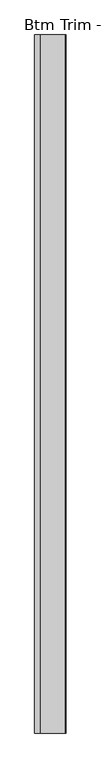
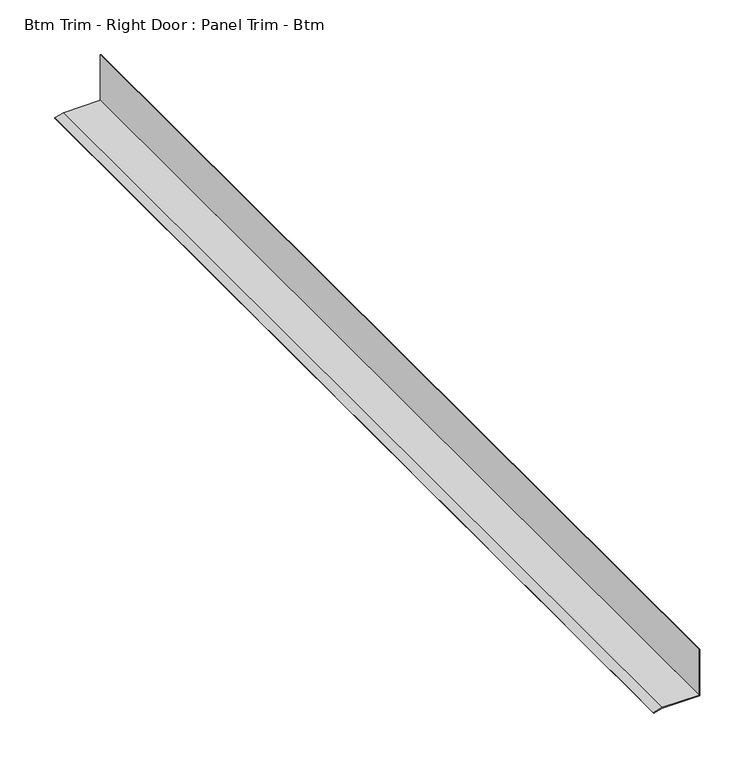
"""IFC4 building model written with IfcOpenShell, lengths in millimetres: proxy geometry, Btm Trim - Right Door : Panel Trim - Btm."""

from ifc_helpers import new_model, si_unit, frame, origin, place, context, project, spatial, polyline, outline, extrude, source, transform, mapped, element, save


def btm_trim_right_door_panel_trim_btm_5f1d7bb7(model_context):
    return source(origin(), model_context, "Body", "SweptSolid", [
        extrude(outline(polyline([(50.8, 587326.1141748), (48.3077022, 587316.8127928), (47.5409986, 587317.0182304), (50.00625, 587326.2186739), (50.00625, 587365.8934739), (101.6, 587365.8934739), (101.6, 587365.1060739), (50.8, 587365.1060739), (50.8, 587326.1141748)])), frame((0.0, -533977.6038841, 0.0), z_axis=(0.0, 1.0, 0.0), x_axis=(0.0, 0.0, 1.0)), (0.0, 0.0, 1.0), 1094.5749),
    ])


if __name__ == "__main__":
    model = new_model("IFC4")
    model_context = context("Model", 3, world=origin())
    ifc_project = project(units=[si_unit("LENGTHUNIT", "METRE", prefix="MILLI")], contexts=[model_context])
    site = spatial("IfcSite", under=ifc_project)
    building = spatial("IfcBuilding", under=site)
    placement = place(None, origin())
    btm_trim_right_door_panel_trim_btm_shape = btm_trim_right_door_panel_trim_btm_5f1d7bb7(model_context)
    element("IfcBuildingElementProxy", 1, Name="Btm Trim - Right Door : Panel Trim - Btm", ObjectType="Btm Trim - Right Door : Panel Trim - Btm", at=placement, inside=building, context=model_context, shape_type="MappedRepresentation", body=[
        mapped(btm_trim_right_door_panel_trim_btm_shape, transform((0.0, 0.0, 0.0), x_axis=(1.0, 0.0, 0.0), y_axis=(0.0, 1.0, 0.0), z_axis=(0.0, 0.0, 1.0))),
    ])
    save(model, "model.ifc")

# Revit data of these elements
# Element 1 (IfcBuildingElementProxy, "Btm Trim - Right Door : Panel Trim - Btm")
#   Materials on its faces: "BASE TRIM BY MTL PANEL MFR."
# Materials
#   "BASE TRIM BY MTL PANEL MFR.": class "Generic", colour RGB 239 242 240, transparency 0, Cost = 0
